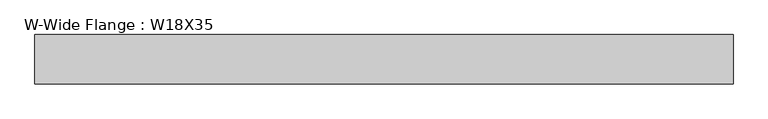
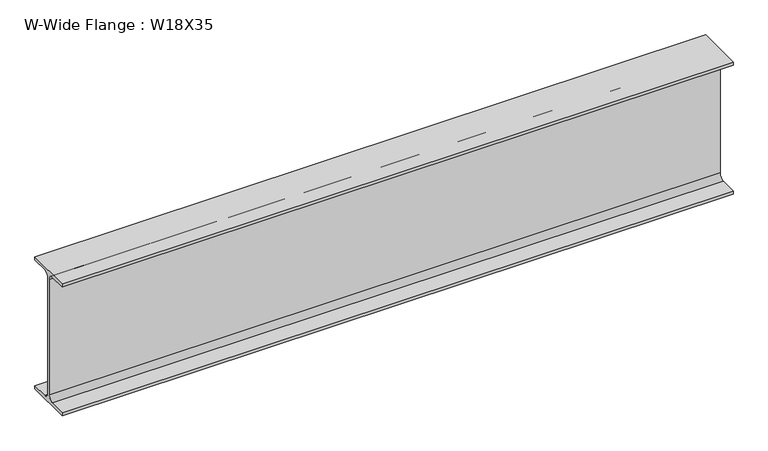
"""IFC4 building model written with IfcOpenShell, lengths in millimetres: beam geometry, W-Wide Flange : W18X35."""

from ifc_helpers import new_model, si_unit, point, frame, frame_2d, origin, place, context, project, spatial, polyline, circle_curve, trimmed, segment, composite_curve, outline, extrude, source, transform, mapped, element, save


def w_wide_flange_w18x35_264b2191(model_context):
    return source(origin(), model_context, "Body", "SweptSolid", [
        extrude(outline(composite_curve([segment(polyline([(76.2, -213.995), (76.2, -224.79), (-76.2, -224.79), (-76.2, -213.995), (-21.59, -213.995)]), True, "CONTINUOUS"), segment(trimmed(circle_curve(frame_2d((-21.59, -196.215)), 17.78), [point((-21.59, -213.995))], [point((-3.81, -196.215))], True, "CARTESIAN"), True, "CONTINUOUS"), segment(polyline([(-3.81, -196.215), (-3.81, 196.215)]), True, "CONTINUOUS"), segment(trimmed(circle_curve(frame_2d((-21.59, 196.215)), 17.78), [point((-3.81, 196.215))], [point((-21.59, 213.995))], True, "CARTESIAN"), True, "CONTINUOUS"), segment(polyline([(-21.59, 213.995), (-76.2, 213.995), (-76.2, 224.79), (76.2, 224.79), (76.2, 213.995), (21.59, 213.995)]), True, "CONTINUOUS"), segment(trimmed(circle_curve(frame_2d((21.59, 196.215)), 17.78), [point((21.59, 213.995))], [point((3.81, 196.215))], True, "CARTESIAN"), True, "CONTINUOUS"), segment(polyline([(3.81, 196.215), (3.81, -196.215)]), True, "CONTINUOUS"), segment(trimmed(circle_curve(frame_2d((21.59, -196.215)), 17.78), [point((3.81, -196.215))], [point((21.59, -213.995))], True, "CARTESIAN"), True, "CONTINUOUS"), segment(polyline([(21.59, -213.995), (76.2, -213.995)]), True, "CONTINUOUS")], self_intersect=False)), frame((-1066.8, 0.0, 0.0), z_axis=(1.0, 0.0, 0.0), x_axis=(0.0, 1.0, 0.0)), (0.0, 0.0, 1.0), 2159.0),
    ])


if __name__ == "__main__":
    model = new_model("IFC4")
    model_context = context("Model", 3, world=origin())
    ifc_project = project(units=[si_unit("LENGTHUNIT", "METRE", prefix="MILLI")], contexts=[model_context])
    site = spatial("IfcSite", under=ifc_project)
    building = spatial("IfcBuilding", under=site)
    placement = place(None, origin())
    w_wide_flange_w18x35_shape = w_wide_flange_w18x35_264b2191(model_context)
    element("IfcBeam", 1, ObjectType="W-Wide Flange : W18X35", at=placement, inside=building, context=model_context, shape_type="MappedRepresentation", body=[
        mapped(w_wide_flange_w18x35_shape, transform((0.0, 0.0, 0.0), x_axis=(1.0, 0.0, 0.0), y_axis=(0.0, 1.0, 0.0), z_axis=(0.0, 0.0, 1.0))),
    ])
    save(model, "model.ifc")

# Revit data of these elements
# Type "W-Wide Flange : W18X35"
#   Assembly Code = "B10"
#   W = 35
#   Length [instance default] = 5' - 0"
#   bf = 0' - 6"
#   d = 1' - 5.7"
#   k = 0' - 1 1/8"
#   k2 = 0' - 0.7"
#   tf = 0' - 0.425"
#   tw = 0' - 0.3"
#   A = 0.0715278 SF
#   Structural Material [instance default] = Steel ASTM A992
# Element 1 (IfcBeam, "W-Wide Flange : W18X35")
#   Structural Material = Steel ASTM A36
#   Materials on its faces: "Steel ASTM A36"
# Materials
#   "Steel ASTM A992": class "Metal", colour RGB 199 199 199, transparency 0, Description = "Structural steel 50ksi", Cost = 0
#   "Steel ASTM A36": class "Metal", colour RGB 199 199 199, transparency 0, Description = "Structural steel, ASTM A36 Grade B, mill finish", Cost = 0
